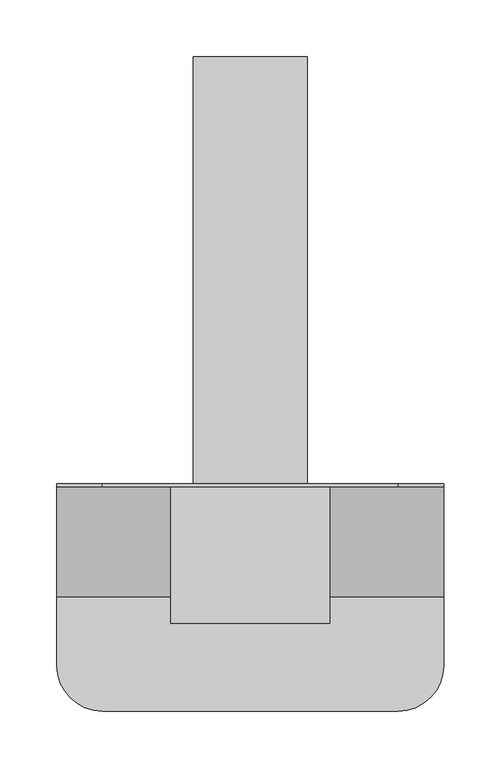
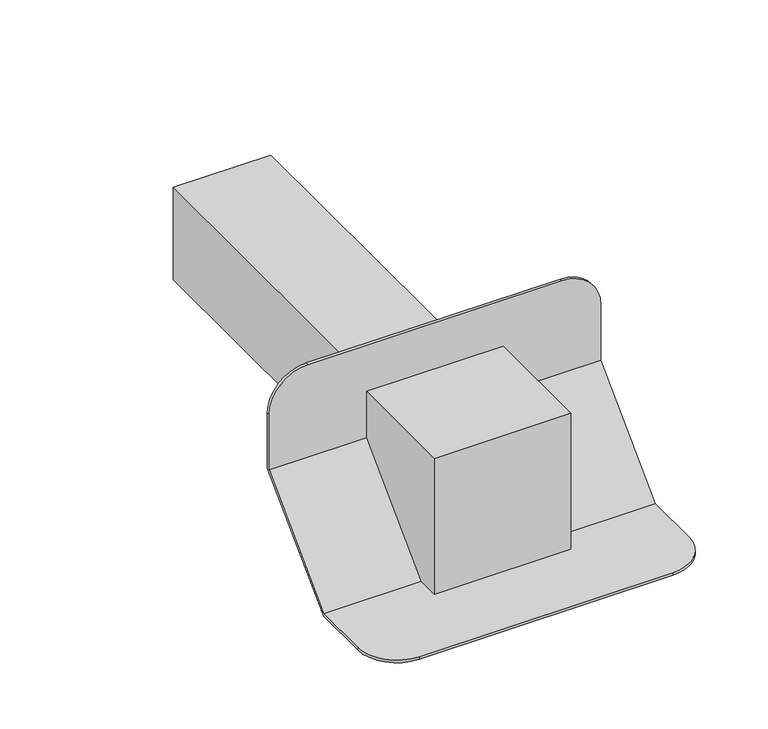
"""IFC4 building model written with IfcOpenShell, lengths in millimetres: proxy geometry, TN_Воронка парапетная ТехноНИКОЛЬ квадратная_Тип 2 : Воронка парапетная ТехноНИКОЛЬ квадратного сечения с галтелью 100х100х600."""

from ifc_helpers import new_model, si_unit, frame, origin, place, context, project, spatial, polyline, circle_curve, outline, extrude, source, transform, mapped, element, save
from ifc_brep_helpers import plane_surface, cylinder_surface, advanced_brep


def specialty_equipment_b9d42960(model_context):
    return source(origin(), model_context, "Body", "SolidModel", [
        extrude(outline(polyline([(-123.0, 150.0), (-3.0, 150.0), (-3.0, 97.0), (-100.0, 0.0), (-123.0, 0.0), (-123.0, 150.0)])), frame((-70.0, 0.0, 0.0), z_axis=(1.0, 0.0, 0.0), x_axis=(0.0, 1.0, 0.0)), (0.0, 0.0, 1.0), 140.0),
        advanced_brep(
        [(50.0, 375.0, 35.0), (-50.0, 375.0, 35.0), (-50.0, 375.0, 135.0), (50.0, 375.0, 135.0), (47.0, 375.0, 38.0), (47.0, 375.0, 132.0), (-47.0, 375.0, 132.0), (-47.0, 375.0, 38.0), (50.0, 0.0, 135.0), (50.0, 0.0, 100.0), (50.0, -65.0, 35.0), (-50.0, 0.0, 135.0), (-50.0, -65.0, 35.0), (-50.0, 0.0, 100.0), (-47.0, -65.0, 38.0), (47.0, -65.0, 38.0), (-47.0, -3.0, 132.0), (-47.0, -3.0, 100.0), (47.0, -3.0, 132.0), (47.0, -3.0, 100.0), (170.0, -3.0, 100.0), (170.0, -3.0, 160.0), (130.0, -3.0, 200.0), (-130.0, -3.0, 200.0), (-170.0, -3.0, 160.0), (-170.0, -3.0, 100.0), (-170.0, 0.0, 100.0), (-170.0, 0.0, 160.0), (-130.0, 0.0, 200.0), (130.0, 0.0, 200.0), (170.0, 0.0, 160.0), (170.0, 0.0, 100.0), (170.0, -100.0, 3.0), (170.0, -160.0, 3.0), (170.0, -160.0, 0.0), (170.0, -100.0, 0.0), (-170.0, -100.0, 0.0), (-170.0, -160.0, 0.0), (-170.0, -160.0, 3.0), (-170.0, -100.0, 3.0), (-130.0, -200.0, 3.0), (130.0, -200.0, 3.0), (130.0, -200.0, 0.0), (-130.0, -200.0, 0.0)],
        [
            (0, 1),
            (1, 2),
            (2, 3),
            (3, 0),
            (4, 5),
            (5, 6),
            (6, 7),
            (7, 4),
            (3, 8),
            (8, 9),
            (9, 10),
            (10, 0),
            (2, 11),
            (11, 8),
            (1, 12),
            (12, 13),
            (13, 11),
            (10, 12),
            (7, 14),
            (14, 15),
            (15, 4),
            (6, 16),
            (16, 17),
            (17, 14),
            (5, 18),
            (18, 16),
            (15, 19),
            (19, 18),
            (20, 21),
            (21, 22, circle_curve(frame((130.0, -3.0, 160.0), z_axis=(0.0, -1.0, 0.0), x_axis=(1.0, 0.0, 0.0)), 40.0)),
            (22, 23),
            (23, 24, circle_curve(frame((-130.0, -3.0, 160.0), z_axis=(0.0, -1.0, 0.0), x_axis=(1.0, 0.0, 0.0)), 40.0)),
            (24, 25),
            (25, 17),
            (19, 20),
            (26, 27),
            (27, 28, circle_curve(frame((-130.0, 0.0, 160.0), z_axis=(0.0, 1.0, 0.0), x_axis=(1.0, 0.0, 0.0)), 40.0)),
            (28, 29),
            (29, 30, circle_curve(frame((130.0, 0.0, 160.0), z_axis=(0.0, 1.0, 0.0), x_axis=(1.0, 0.0, 0.0)), 40.0)),
            (30, 31),
            (31, 9),
            (13, 26),
            (20, 32),
            (32, 33),
            (33, 34),
            (34, 35),
            (35, 31),
            (30, 21),
            (29, 22),
            (28, 23),
            (27, 24),
            (26, 36),
            (36, 37),
            (37, 38),
            (38, 39),
            (39, 25),
            (32, 39),
            (38, 40, circle_curve(frame((-130.0, -160.0, 3.0), z_axis=(0.0, 0.0, 1.0), x_axis=(1.0, 0.0, 0.0)), 40.0)),
            (40, 41),
            (41, 33, circle_curve(frame((130.0, -160.0, 3.0), z_axis=(0.0, 0.0, 1.0), x_axis=(1.0, 0.0, 0.0)), 40.0)),
            (34, 42, circle_curve(frame((130.0, -160.0, 0.0), z_axis=(0.0, 0.0, -1.0), x_axis=(1.0, 0.0, 0.0)), 40.0)),
            (42, 43),
            (43, 37, circle_curve(frame((-130.0, -160.0, 0.0), z_axis=(0.0, 0.0, -1.0), x_axis=(1.0, 0.0, 0.0)), 40.0)),
            (36, 35),
            (43, 40),
            (42, 41),
        ],
        [
            plane_surface(frame((50.0, 375.0, 35.0), z_axis=(0.0, 1.0, 0.0), x_axis=(0.0, 0.0, -1.0))),
            plane_surface(frame((50.0, -100.0, 35.0), z_axis=(1.0, 0.0, 0.0), x_axis=(0.0, 1.0, 0.0))),
            plane_surface(frame((50.0, -100.0, 135.0), z_axis=(0.0, 0.0, 1.0), x_axis=(0.0, 1.0, 0.0))),
            plane_surface(frame((-50.0, -100.0, 135.0), z_axis=(-1.0, 0.0, 0.0), x_axis=(0.0, 1.0, 0.0))),
            plane_surface(frame((-50.0, -100.0, 35.0), z_axis=(0.0, 0.0, -1.0), x_axis=(0.0, 1.0, 0.0))),
            plane_surface(frame((47.0, -100.0, 38.0), z_axis=(0.0, 0.0, 1.0), x_axis=(0.0, 1.0, 0.0))),
            plane_surface(frame((-47.0, -100.0, 38.0), z_axis=(1.0, 0.0, 0.0), x_axis=(0.0, 1.0, 0.0))),
            plane_surface(frame((-47.0, -100.0, 132.0), z_axis=(0.0, 0.0, -1.0), x_axis=(0.0, 1.0, 0.0))),
            plane_surface(frame((47.0, -100.0, 132.0), z_axis=(-1.0, 0.0, 0.0), x_axis=(0.0, 1.0, 0.0))),
            plane_surface(frame((170.0, -3.0, 160.0), z_axis=(0.0, -1.0, 0.0), x_axis=(0.0, 0.0, 1.0))),
            plane_surface(frame((170.0, 0.0, 160.0), z_axis=(0.0, 1.0, 0.0), x_axis=(0.0, 0.0, -1.0))),
            plane_surface(frame((170.0, -3.0, 100.0), z_axis=(1.0, 0.0, 0.0), x_axis=(0.0, 1.0, 0.0))),
            cylinder_surface(frame((130.0, 0.0, 160.0), z_axis=(0.0, -1.0, 0.0), x_axis=(1.0, 0.0, 0.0)), 40.0),
            plane_surface(frame((130.0, -3.0, 200.0), z_axis=(0.0, 0.0, 1.0), x_axis=(0.0, 1.0, 0.0))),
            cylinder_surface(frame((-130.0, 0.0, 160.0), z_axis=(0.0, -1.0, 0.0), x_axis=(1.0, 0.0, 0.0)), 40.0),
            plane_surface(frame((-170.0, -3.0, 160.0), z_axis=(-1.0, 0.0, 0.0), x_axis=(0.0, 1.0, 0.0))),
            plane_surface(frame((170.0, 0.0, 3.0), z_axis=(0.0, 0.0, 1.0), x_axis=(0.0, 1.0, 0.0))),
            plane_surface(frame((170.0, 0.0, 0.0), z_axis=(0.0, 0.0, -1.0), x_axis=(0.0, -1.0, 0.0))),
            cylinder_surface(frame((-130.0, -160.0, 0.0), z_axis=(0.0, 0.0, 1.0), x_axis=(1.0, 0.0, 0.0)), 40.0),
            plane_surface(frame((-130.0, -200.0, 3.0), z_axis=(0.0, -1.0, 0.0), x_axis=(0.0, 0.0, -1.0))),
            cylinder_surface(frame((130.0, -160.0, 0.0), z_axis=(0.0, 0.0, 1.0), x_axis=(1.0, 0.0, 0.0)), 40.0),
            plane_surface(frame((170.0, -3.0, 100.0), z_axis=(0.0, -0.7071067811865469, 0.7071067811865481), x_axis=(-1.0, 0.0, 0.0))),
            plane_surface(frame((170.0, -100.0, 0.0), z_axis=(0.0, 0.7071067811865468, -0.7071067811865482), x_axis=(-1.0, 0.0, 0.0))),
        ],
        [
            (0, [[1, 2, 3, 4], [5, 6, 7, 8]]),
            (1, [[-4, 9, 10, 11, 12]]),
            (2, [[-3, 13, 14, -9]]),
            (3, [[-2, 15, 16, 17, -13]]),
            (4, [[-1, -12, 18, -15]]),
            (5, [[-8, 19, 20, 21]]),
            (6, [[-19, -7, 22, 23, 24]]),
            (7, [[-22, -6, 25, 26]]),
            (8, [[-25, -5, -21, 27, 28]]),
            (9, [[29, 30, 31, 32, 33, 34, -23, -26, -28, 35]]),
            (10, [[36, 37, 38, 39, 40, 41, -10, -14, -17, 42]]),
            (11, [[-29, 43, 44, 45, 46, 47, -40, 48]]),
            (12, [[-30, -48, -39, 49]]),
            (13, [[-31, -49, -38, 50]]),
            (14, [[-32, -50, -37, 51]]),
            (15, [[-33, -51, -36, 52, 53, 54, 55, 56]]),
            (16, [[-44, 57, -55, 58, 59, 60]]),
            (17, [[61, 62, 63, -53, 64, -46]]),
            (18, [[-58, -54, -63, 65]]),
            (19, [[-59, -65, -62, 66]]),
            (20, [[-60, -66, -61, -45]]),
            (21, [[-43, -35, -27, -20, -24, -34, -56, -57]]),
            (22, [[-47, -64, -52, -42, -16, -18, -11, -41]]),
        ],
    ),
    ])


if __name__ == "__main__":
    model = new_model("IFC4")
    model_context = context("Model", 3, world=origin())
    ifc_project = project(units=[si_unit("LENGTHUNIT", "METRE", prefix="MILLI")], contexts=[model_context])
    site = spatial("IfcSite", under=ifc_project)
    building = spatial("IfcBuilding", under=site)
    placement = place(None, origin())
    specialty_equipment_shape = specialty_equipment_b9d42960(model_context)
    element("IfcBuildingElementProxy", 1, Name="TN_Воронка парапетная ТехноНИКОЛЬ квадратная_Тип 2 : Воронка парапетная ТехноНИКОЛЬ квадратного сечения с галтелью 100х100х600", ObjectType="TN_Воронка парапетная ТехноНИКОЛЬ квадратная_Тип 2 : Воронка парапетная ТехноНИКОЛЬ квадратного сечения с галтелью 100х100х600", at=placement, inside=building, context=model_context, shape_type="MappedRepresentation", body=[
        mapped(specialty_equipment_shape, transform((0.0, 0.0, 0.0), x_axis=(1.0, 0.0, 0.0), y_axis=(0.0, 1.0, 0.0), z_axis=(0.0, 0.0, 1.0))),
    ])
    save(model, "model.ifc")

# Revit data of these elements
# Type "TN_Воронка парапетная ТехноНИКОЛЬ квадратная_Тип 2 : Воронка парапетная ТехноНИКОЛЬ квадратного сечения с галтелью 100х100х600"
#   Description = "Воронка предназначена для организации внешнего водостока через балконы и парапеты на пониженных участках кровли. Также воронка может являться парапетным переливом, которая устанавливается в случаях аварийного сброса воды при засорении основной воронки внутреннего водостока. Воронки комплектуются листвоуловителем и имеют сформированную галтель размером 100ммх100мм, что облегчает монтаж битумной гидроизоляции в данном узле и повышает его надежность при эксплуатации.\r\nСоединение с водосточной системой осуществляется через отвод угловой, с квадратного сечения в круглое"
#   Manufacturer = "ТехноНИКОЛЬ"
#   ADSK_Примечание = ""
#   ADSK_Обозначение = "ТехноНИКОЛЬ"
#   ADSK_Наименование = "Воронка парапетная ТехноНИКОЛЬ квадратного сечения с галтелью 100х100х600"
#   ADSK_Марка = ""
#   ADSK_Код изделия = "69751"
#   ADSK_Завод-изготовитель = "ТехноНИКОЛЬ"
#   ADSK_Единица измерения = "шт."
#   ADSK_Группирование = "Комплектующие и воронки"
#   ADSK_URL страницы изделия = ""
#   ADSK_URL документации изделия = ""
#   Ширина фланца = 340 mm
#   Размер фланца по вертикали = 200 mm
#   Длина расчетная [instance default] = 375 mm
#   Длина отвода [instance default] = 375 mm
#   Размер фланца по горизонтали = 200 mm
#   ADSK_Количество = 1
#   Видимость_Переход [instance default] = no
#   Видимость_Листоуловитель [instance default] = no
#   Материал = TN_ПВХ_Черный
#   Default Elevation = 0
#   URL = ""
# Element 1 (IfcBuildingElementProxy, "TN_Воронка парапетная ТехноНИКОЛЬ квадратная_Тип 2 : Воронка парапетная ТехноНИКОЛЬ квадратного сечения с галтелью 100х100х600")
#   Видимость_Переход = yes
#   Видимость_Листоуловитель = yes
#   Materials on its faces: "TN_ПВХ_Черный"
# Materials
#   "TN_ПВХ_Черный": class "Типовые", colour RGB 48 48 48, transparency 0, Cost = 0
